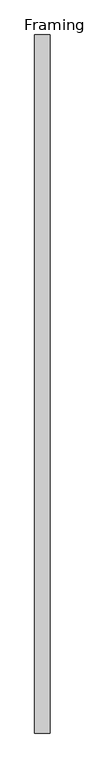
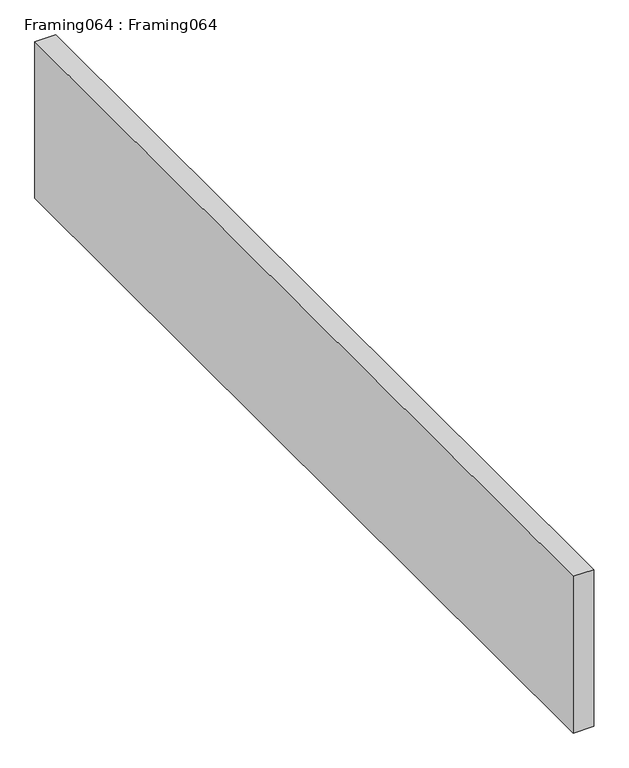
"""IFC4 building model written with IfcOpenShell, lengths in millimetres: proxy geometry, Framing064 : Framing064."""

from ifc_helpers import new_model, si_unit, frame, origin, place, context, project, spatial, polyline, outline, extrude, source, transform, mapped, element, save


def framing064_framing064_83d7daf7(model_context):
    return source(origin(), model_context, "Body", "SweptSolid", [
        extrude(outline(polyline([(-2406.6602963, -1052.8906574), (-2451.1102963, -1052.8906574), (-2451.1102963, 947.1093426), (-2406.6602963, 947.1093426), (-2406.6602963, -1052.8906574)])), frame((0.0, 0.0, 42133.8036692), z_axis=(0.0, 0.0, 1.0), x_axis=(1.0, 0.0, 0.0)), (0.0, 0.0, 1.0), 355.2981173),
    ])


if __name__ == "__main__":
    model = new_model("IFC4")
    model_context = context("Model", 3, world=origin())
    ifc_project = project(units=[si_unit("LENGTHUNIT", "METRE", prefix="MILLI")], contexts=[model_context])
    site = spatial("IfcSite", under=ifc_project)
    building = spatial("IfcBuilding", under=site)
    placement = place(None, origin())
    framing064_framing064_shape = framing064_framing064_83d7daf7(model_context)
    element("IfcBuildingElementProxy", 1, Name="Framing064 : Framing064", ObjectType="Framing064 : Framing064", at=placement, inside=building, context=model_context, shape_type="MappedRepresentation", body=[
        mapped(framing064_framing064_shape, transform((0.0, 0.0, 0.0), x_axis=(1.0, 0.0, 0.0), y_axis=(0.0, 1.0, 0.0), z_axis=(0.0, 0.0, 1.0))),
    ])
    save(model, "model.ifc")

# Revit data of these elements
# Type "Framing064 : Framing064"
#   NameOverride = "Framing064"
# Element 1 (IfcBuildingElementProxy, "Framing064 : Framing064")
#   Materials on its faces: "WOOD FRAMING (SEE STRUCT DWGS)"
# Materials
#   "WOOD FRAMING (SEE STRUCT DWGS)": class "Unassigned", colour RGB 224 188 168, transparency 0, Cost = 0
